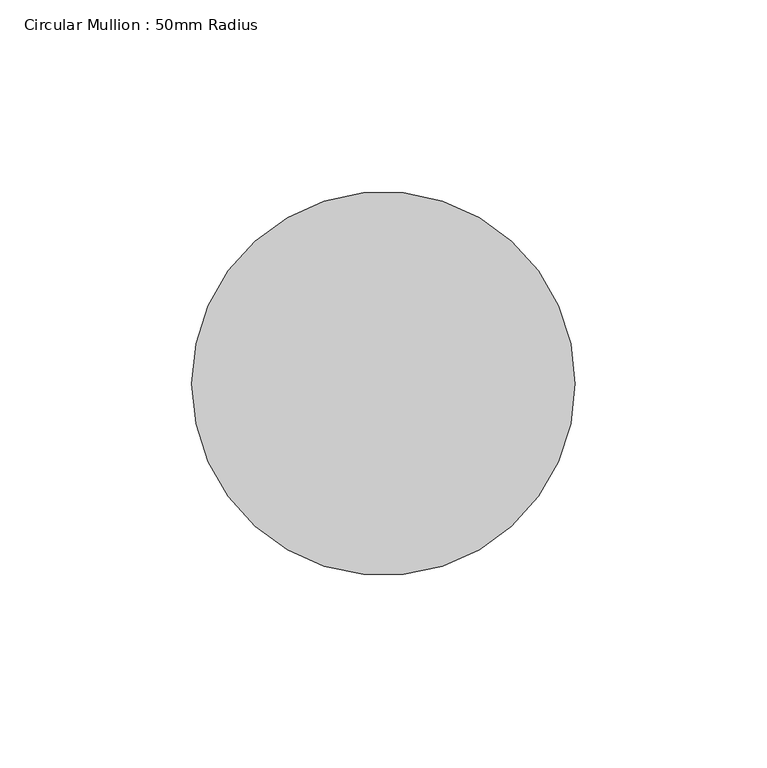
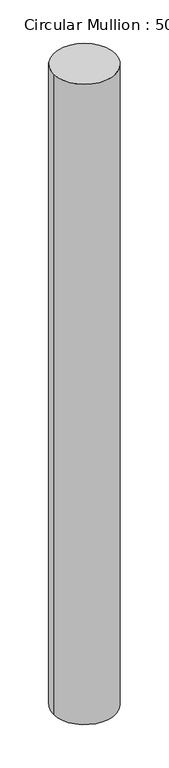
"""IFC4 building model written with IfcOpenShell, lengths in millimetres: member geometry, Circular Mullion : 50mm Radius."""

from ifc_helpers import new_model, si_unit, point, frame, origin, origin_2d, place, context, project, spatial, circle_curve, trimmed, segment, composite_curve, outline, extrude, source, transform, mapped, element, save


def circular_mullion_50mm_radius_0188850a(model_context):
    return source(origin(), model_context, "Body", "SweptSolid", [
        extrude(outline(composite_curve([segment(trimmed(circle_curve(origin_2d(), 50.0), [point((50.0, 0.0))], [point((-50.0, 0.0))], False, "CARTESIAN"), True, "CONTINUOUS"), segment(trimmed(circle_curve(origin_2d(), 50.0), [point((-50.0, 0.0))], [point((50.0, 0.0))], False, "CARTESIAN"), True, "CONTINUOUS")], self_intersect=False)), frame((0.0, 0.0, -1091.4252419), z_axis=(0.0, 0.0, 1.0), x_axis=(1.0, 0.0, 0.0)), (0.0, 0.0, 1.0), 1091.4252419),
    ])


if __name__ == "__main__":
    model = new_model("IFC4")
    model_context = context("Model", 3, world=origin())
    ifc_project = project(units=[si_unit("LENGTHUNIT", "METRE", prefix="MILLI")], contexts=[model_context])
    site = spatial("IfcSite", under=ifc_project)
    building = spatial("IfcBuilding", under=site)
    placement = place(None, origin())
    circular_mullion_50mm_radius_shape = circular_mullion_50mm_radius_0188850a(model_context)
    element("IfcMember", 1, ObjectType="Circular Mullion : 50mm Radius", at=placement, inside=building, context=model_context, shape_type="MappedRepresentation", body=[
        mapped(circular_mullion_50mm_radius_shape, transform((0.0, 0.0, 0.0), x_axis=(1.0, 0.0, 0.0), y_axis=(0.0, 1.0, 0.0), z_axis=(0.0, 0.0, 1.0))),
    ])
    save(model, "model.ifc")

# Revit data of these elements
# Type "Circular Mullion : 50mm Radius"
#   built-in parameter 1007350 = 0.164042 (stored number, unit not read)
# Element 1 (IfcMember, "Circular Mullion : 50mm Radius")
#   Materials on its faces: "Aluminium"
# Materials
#   "Aluminium": class "Metal", colour RGB 247 247 247, transparency 0, Description = "Aluminium 6061", Cost = 0
